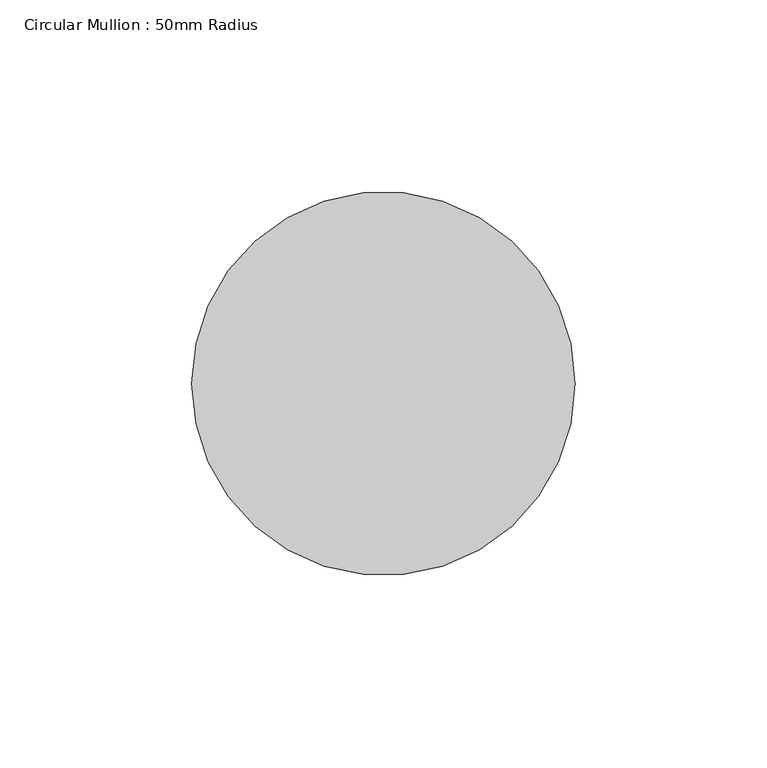
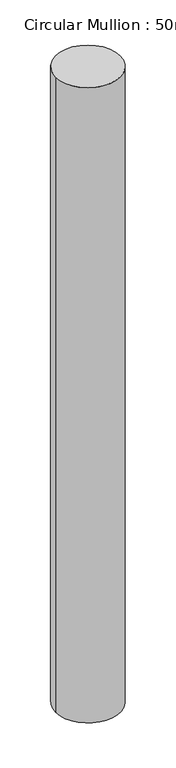
"""IFC4 building model written with IfcOpenShell, lengths in millimetres: member geometry, Circular Mullion : 50mm Radius."""

from ifc_helpers import new_model, si_unit, point, frame, origin, origin_2d, place, context, project, spatial, circle_curve, trimmed, segment, composite_curve, outline, extrude, source, transform, mapped, element, save


def circular_mullion_50mm_radius_63f0b049(model_context):
    return source(origin(), model_context, "Body", "SweptSolid", [
        extrude(outline(composite_curve([segment(trimmed(circle_curve(origin_2d(), 50.0), [point((50.0, 0.0))], [point((-50.0, 0.0))], False, "CARTESIAN"), True, "CONTINUOUS"), segment(trimmed(circle_curve(origin_2d(), 50.0), [point((-50.0, 0.0))], [point((50.0, 0.0))], False, "CARTESIAN"), True, "CONTINUOUS")], self_intersect=False)), frame((0.0, 0.0, -1041.0593481), z_axis=(0.0, 0.0, 1.0), x_axis=(1.0, 0.0, 0.0)), (0.0, 0.0, 1.0), 1041.0593481),
    ])


if __name__ == "__main__":
    model = new_model("IFC4")
    model_context = context("Model", 3, world=origin())
    ifc_project = project(units=[si_unit("LENGTHUNIT", "METRE", prefix="MILLI")], contexts=[model_context])
    site = spatial("IfcSite", under=ifc_project)
    building = spatial("IfcBuilding", under=site)
    placement = place(None, origin())
    circular_mullion_50mm_radius_shape = circular_mullion_50mm_radius_63f0b049(model_context)
    element("IfcMember", 1, ObjectType="Circular Mullion : 50mm Radius", at=placement, inside=building, context=model_context, shape_type="MappedRepresentation", body=[
        mapped(circular_mullion_50mm_radius_shape, transform((0.0, 0.0, 0.0), x_axis=(1.0, 0.0, 0.0), y_axis=(0.0, 1.0, 0.0), z_axis=(0.0, 0.0, 1.0))),
    ])
    save(model, "model.ifc")

# Revit data of these elements
# Type "Circular Mullion : 50mm Radius"
#   built-in parameter 1007350 = 0.164042 (stored number, unit not read)
# Element 1 (IfcMember, "Circular Mullion : 50mm Radius")
#   Materials on its faces: "Aluminium"
# Materials
#   "Aluminium": class "Metal", colour RGB 247 247 247, transparency 0, Description = "Aluminium 6061", Cost = 0
